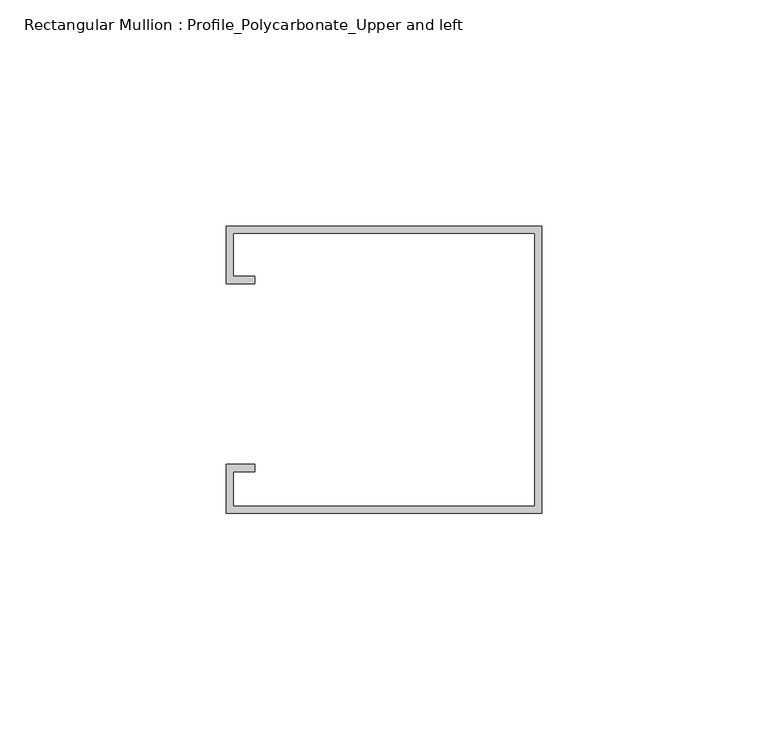
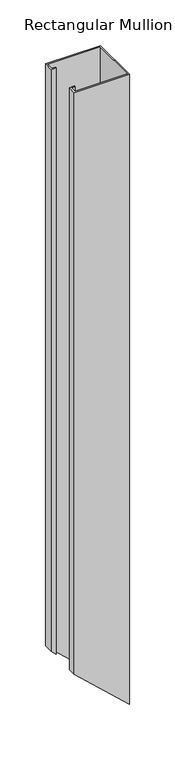
"""IFC4 building model written with IfcOpenShell, lengths in millimetres: member geometry, Rectangular Mullion : Profile_Polycarbonate_Upper and left."""

from ifc_helpers import new_model, si_unit, origin, place, context, project, spatial, faceted_brep, source, transform, mapped, element, save


def rectangular_mullion_profile_polycarbonate_upper_and_left_1f329f0a(model_context):
    return source(origin(), model_context, "Body", "Brep", [
        faceted_brep([(0.0, 32.7, 0.0), (-69.85, 32.7, 0.0), (-69.85, 20.0, 0.0), (-63.5, 20.0, 0.0), (-63.5, 21.5875, 0.0), (-68.2625, 21.5875, 0.0), (-68.2625, 31.1125, 0.0), (-1.5875, 31.1125, 0.0), (-1.5875, -29.2125, 0.0), (-68.2625, -29.2125, 0.0), (-68.2625, -21.5875, 0.0), (-63.5, -21.5875, 0.0), (-63.5, -20.0, 0.0), (-69.85, -20.0, 0.0), (-69.85, -30.8, 0.0), (0.0, -30.8, 0.0), (0.0, 32.7, -844.0208333), (-69.85, 32.7, -779.7495516), (-69.85, 20.0, -779.7495516), (-63.5, 20.0, -785.5923954), (-63.5, 21.5875, -785.5923954), (-68.2625, 21.5875, -781.2102625), (-68.2625, 31.1125, -781.2102625), (-1.5875, 31.1125, -842.5601224), (-1.5875, -29.2125, -842.5601224), (-68.2625, -29.2125, -781.2102625), (-68.2625, -21.5875, -781.2102625), (-63.5, -21.5875, -785.5923954), (-63.5, -20.0, -785.5923954), (-69.85, -20.0, -779.7495516), (-69.85, -30.8, -779.7495516), (0.0, -30.8, -844.0208333)], [[[0, 1, 2, 3, 4, 5, 6, 7, 8, 9, 10, 11, 12, 13, 14, 15]], [[1, 0, 16, 17]], [[2, 1, 17, 18]], [[3, 2, 18, 19]], [[4, 3, 19, 20]], [[5, 4, 20, 21]], [[6, 5, 21, 22]], [[7, 6, 22, 23]], [[8, 7, 23, 24]], [[9, 8, 24, 25]], [[10, 9, 25, 26]], [[11, 10, 26, 27]], [[12, 11, 27, 28]], [[13, 12, 28, 29]], [[14, 13, 29, 30]], [[15, 14, 30, 31]], [[0, 15, 31, 16]], [[16, 31, 30, 29, 28, 27, 26, 25, 24, 23, 22, 21, 20, 19, 18, 17]]]),
    ])


if __name__ == "__main__":
    model = new_model("IFC4")
    model_context = context("Model", 3, world=origin())
    ifc_project = project(units=[si_unit("LENGTHUNIT", "METRE", prefix="MILLI")], contexts=[model_context])
    site = spatial("IfcSite", under=ifc_project)
    building = spatial("IfcBuilding", under=site)
    placement = place(None, origin())
    rectangular_mullion_profile_polycarbonate_upper_and_left_shape = rectangular_mullion_profile_polycarbonate_upper_and_left_1f329f0a(model_context)
    element("IfcMember", 1, ObjectType="Rectangular Mullion : Profile_Polycarbonate_Upper and left", at=placement, inside=building, context=model_context, shape_type="MappedRepresentation", body=[
        mapped(rectangular_mullion_profile_polycarbonate_upper_and_left_shape, transform((0.0, 0.0, 0.0), x_axis=(1.0, 0.0, 0.0), y_axis=(0.0, 1.0, 0.0), z_axis=(0.0, 0.0, 1.0))),
    ])
    save(model, "model.ifc")

# Revit data of these elements
# Type "Rectangular Mullion : Profile_Polycarbonate_Upper and left"
#   built-in parameter 1007322 = 0.208333 (stored number, unit not read)
#   built-in parameter 1007321 = 0.00520833 (stored number, unit not read)
#   built-in parameter 1007320 = 0 (stored number, unit not read)
# Element 1 (IfcMember, "Rectangular Mullion : Profile_Polycarbonate_Upper and left")
#   Materials on its faces: "ALUMINUM PROFILE AT POLYCARBONATE PANEL"
# Materials
#   "ALUMINUM PROFILE AT POLYCARBONATE PANEL": class "Metal", colour RGB 244 244 244, transparency 0, Description = "Aluminum 6061", Cost = 0
